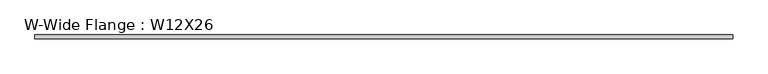
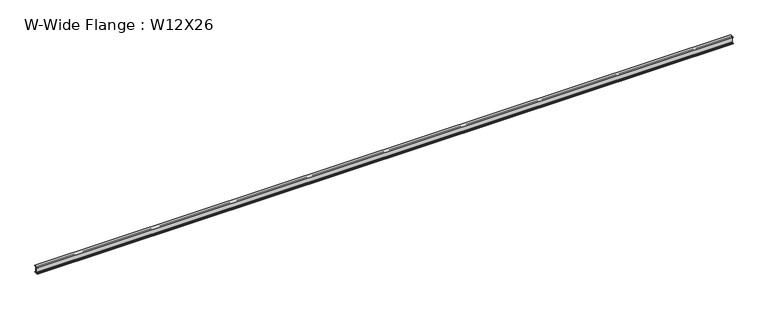
"""IFC4 building model written with IfcOpenShell, lengths in millimetres: beam geometry, W-Wide Flange : W12X26."""

import ifcopenshell
import ifcopenshell.guid

model = None  # the IFC model being written
_history = None  # IfcOwnerHistory: only IFC2X3 demands one
_inside = {}  # id of a spatial element -> (the spatial element, [elements in it])
_under = {}  # id of a project, library or spatial element -> (it, [spatial elements below it])
_declared = {}  # id of a project -> (the project, [libraries it declares])
_typed = {}  # id of a type object -> (the type object, [elements of that type])
_made_of = {}  # id of a material, layer set ... -> (it, [elements and type objects made of it])


def new_model(schema):
    """Start an empty IFC model of exactly this schema.

    Asked for "IFC4X3", IfcOpenShell would pick the latest addendum, in which some entities
    have other attributes; the version numbers below select the first issue.
    IFC2X3 requires an IfcOwnerHistory on every rooted entity: one is made here for all.
    """
    global model, _history
    if schema == "IFC4X3":
        model = ifcopenshell.file(schema_version=(4, 3, 0, 0))
    else:
        model = ifcopenshell.file(schema=schema)
    _inside.clear()
    _under.clear()
    _declared.clear()
    _typed.clear()
    _made_of.clear()
    _history = None
    if model.schema == "IFC2X3":
        org = make("IfcOrganization", Name="unknown")
        user = make(
            "IfcPersonAndOrganization",
            ThePerson=make("IfcPerson", FamilyName="unknown"),
            TheOrganization=org,
        )
        app = make(
            "IfcApplication",
            ApplicationDeveloper=org,
            Version="unknown",
            ApplicationFullName="unknown",
            ApplicationIdentifier="unknown",
        )
        _history = make(
            "IfcOwnerHistory",
            OwningUser=user,
            OwningApplication=app,
            ChangeAction="ADDED",
            CreationDate=0,
        )
    return model


def make(cls, **values):
    """One entity of the class cls with the attributes given. An attribute that is None is left unset."""
    return model.create_entity(
        cls, **{name: value for name, value in values.items() if value is not None}
    )


def rooted(cls, **values):
    """An entity with a GlobalId (a new one), such as an element, a storey or a relation."""
    return make(cls, GlobalId=ifcopenshell.guid.new(), OwnerHistory=_history, **values)


def si_unit(unit_type, name, prefix=None):
    """IfcSIUnit, for example si_unit("LENGTHUNIT", "METRE", prefix="MILLI")."""
    return make("IfcSIUnit", UnitType=unit_type, Prefix=prefix, Name=name)


def assignment(units):
    """IfcUnitAssignment: the units of a project."""
    return None if units is None else make("IfcUnitAssignment", Units=units)


def point(xyz):
    """IfcCartesianPoint."""
    return None if xyz is None else make("IfcCartesianPoint", Coordinates=xyz)


def direction(xyz):
    """IfcDirection."""
    return None if xyz is None else make("IfcDirection", DirectionRatios=xyz)


def frame(location, z_axis=None, x_axis=None):
    """IfcAxis2Placement3D, a coordinate frame: its origin and axes. An axis left out is left unset."""
    return make(
        "IfcAxis2Placement3D",
        Location=point(location),
        Axis=direction(z_axis),
        RefDirection=direction(x_axis),
    )


def frame_2d(location, x_axis=None):
    """IfcAxis2Placement2D, a coordinate frame in the plane: its origin and x axis."""
    return make(
        "IfcAxis2Placement2D", Location=point(location), RefDirection=direction(x_axis)
    )


def origin():
    """The frame at (0, 0, 0) with its axes left unset."""
    return frame((0.0, 0.0, 0.0))


def place(relative_to, where):
    """IfcLocalPlacement: puts the frame where relative to a parent placement (None: the world)."""
    return make(
        "IfcLocalPlacement", PlacementRelTo=relative_to, RelativePlacement=where
    )


def context(
    kind, dimensions, precision=None, world=None, true_north=None, identifier=None
):
    """IfcGeometricRepresentationContext, for example the 3D "Model" context."""
    return make(
        "IfcGeometricRepresentationContext",
        ContextIdentifier=identifier,
        ContextType=kind,
        CoordinateSpaceDimension=dimensions,
        Precision=precision,
        WorldCoordinateSystem=world,
        TrueNorth=true_north,
    )


def project(units=None, contexts=None):
    """IfcProject with its units and contexts."""
    return rooted(
        "IfcProject",
        Name="project",
        RepresentationContexts=contexts,
        UnitsInContext=assignment(units),
    )


def spatial(cls, under=None, at=None, **own):
    """A site, building, storey or space (cls), placed at a placement, below another one or the project."""
    s = rooted(cls, ObjectPlacement=at, **own)
    if under is not None:
        _under.setdefault(under.id(), (under, []))[1].append(s)
    return s


def polyline(points):
    """IfcPolyline through the points."""
    return make("IfcPolyline", Points=[point(p) for p in points])


def circle_curve(where, radius):
    """IfcCircle in the frame where."""
    return make("IfcCircle", Position=where, Radius=radius)


def trimmed(basis, trim1, trim2, sense, master):
    """IfcTrimmedCurve: the piece of a basis curve between two trims."""
    return make(
        "IfcTrimmedCurve",
        BasisCurve=basis,
        Trim1=trim1,
        Trim2=trim2,
        SenseAgreement=sense,
        MasterRepresentation=master,
    )


def segment(curve, same_sense, transition):
    """IfcCompositeCurveSegment."""
    return make(
        "IfcCompositeCurveSegment",
        Transition=transition,
        SameSense=same_sense,
        ParentCurve=curve,
    )


def composite_curve(segments, self_intersect=None):
    """IfcCompositeCurve: segments joined end to end."""
    return make("IfcCompositeCurve", Segments=segments, SelfIntersect=self_intersect)


def outline(outer, holes=None, kind="AREA"):
    """IfcArbitraryClosedProfileDef: a profile drawn as a closed curve; with holes, ...WithVoids."""
    if holes is None:
        return make("IfcArbitraryClosedProfileDef", ProfileType=kind, OuterCurve=outer)
    return make(
        "IfcArbitraryProfileDefWithVoids",
        ProfileType=kind,
        OuterCurve=outer,
        InnerCurves=holes,
    )


def extrude(swept, where, along, depth):
    """IfcExtrudedAreaSolid: the profile swept, set in the frame where, extruded along a direction by depth."""
    return make(
        "IfcExtrudedAreaSolid",
        SweptArea=swept,
        Position=where,
        ExtrudedDirection=direction(along),
        Depth=depth,
    )


def shape(context_of_items, identifier, shape_type, items):
    """IfcShapeRepresentation: the items that make up one representation, for example the "Body"."""
    return make(
        "IfcShapeRepresentation",
        ContextOfItems=context_of_items,
        RepresentationIdentifier=identifier,
        RepresentationType=shape_type,
        Items=items,
    )


def source(mapping_origin, context_of_items, identifier, shape_type, items):
    """IfcRepresentationMap: a shape defined once, which mapped items show again and again."""
    return make(
        "IfcRepresentationMap",
        MappingOrigin=mapping_origin,
        MappedRepresentation=shape(context_of_items, identifier, shape_type, items),
    )


def transform(
    local_origin,
    x_axis=None,
    y_axis=None,
    z_axis=None,
    scale=None,
    scale2=None,
    scale3=None,
    uniform=True,
):
    """IfcCartesianTransformationOperator3D, or its non-uniform kind. x_axis, y_axis, z_axis: its Axis1, 2, 3."""
    if uniform:
        return make(
            "IfcCartesianTransformationOperator3D",
            Axis1=direction(x_axis),
            Axis2=direction(y_axis),
            LocalOrigin=point(local_origin),
            Scale=scale,
            Axis3=direction(z_axis),
        )
    return make(
        "IfcCartesianTransformationOperator3DnonUniform",
        Axis1=direction(x_axis),
        Axis2=direction(y_axis),
        LocalOrigin=point(local_origin),
        Scale=scale,
        Axis3=direction(z_axis),
        Scale2=scale2,
        Scale3=scale3,
    )


def mapped(mapping_source, mapping_target):
    """IfcMappedItem: shows the shape of a source again, moved by a transform."""
    return make(
        "IfcMappedItem", MappingSource=mapping_source, MappingTarget=mapping_target
    )


def made_of(thing, what):
    """Note that an element or type object is made of a material, layer set ...; save() writes the relation."""
    if what is not None:
        _made_of.setdefault(what.id(), (what, []))[1].append(thing)
    return thing


def element(
    cls,
    number,
    at=None,
    inside=None,
    cuts=None,
    type_object=None,
    material=None,
    context=None,
    identifier="Body",
    shape_type=None,
    held_by="IfcProductDefinitionShape",
    body=None,
    shapes=None,
    **own,
):
    """One element of the class cls, such as IfcWall. Its Tag is "e" and its number.

    at: its placement. inside: the storey or other place that contains it. cuts: it is an
    opening in that element (IfcRelVoidsElement). A single representation is given by context,
    identifier, shape_type and body (its items); several are given by shapes. held_by: the class
    of the entity that holds the representations. save() writes the other relations.
    """
    e = rooted(cls, Tag="e%d" % number, ObjectPlacement=at, **own)
    if body is not None:
        shapes = [shape(context, identifier, shape_type, body)]
    if shapes is not None:
        e.Representation = make(held_by, Representations=shapes)
    if inside is not None:
        _inside.setdefault(inside.id(), (inside, []))[1].append(e)
    if cuts is not None:
        rooted(
            "IfcRelVoidsElement", RelatingBuildingElement=cuts, RelatedOpeningElement=e
        )
    if type_object is not None:
        _typed.setdefault(type_object.id(), (type_object, []))[1].append(e)
    return made_of(e, material)


def aggregate(whole, parts):
    """IfcRelAggregates: a whole, such as a stair, and the parts it consists of."""
    return rooted("IfcRelAggregates", RelatingObject=whole, RelatedObjects=parts)


def save(model, path):
    """Write the relations noted so far, then the file.

    IfcRelAggregates (storeys below a building ...), IfcRelContainedInSpatialStructure (elements
    in a storey), IfcRelDefinesByType, IfcRelAssociatesMaterial and IfcRelDeclares: one each for
    every whole, place, type object, material and project.
    """
    for whole, parts in _under.values():
        aggregate(whole, parts)
    for where, things in _inside.values():
        rooted(
            "IfcRelContainedInSpatialStructure",
            RelatedElements=things,
            RelatingStructure=where,
        )
    for kind, things in _typed.values():
        rooted("IfcRelDefinesByType", RelatedObjects=things, RelatingType=kind)
    for what, things in _made_of.values():
        rooted("IfcRelAssociatesMaterial", RelatedObjects=things, RelatingMaterial=what)
    for by, libraries in _declared.values():
        rooted("IfcRelDeclares", RelatingContext=by, RelatedDefinitions=libraries)
    model.write(path)


def w_wide_flange_w12x26_ee37c196(model_context):
    return source(origin(), model_context, "Body", "SweptSolid", [
        extrude(outline(composite_curve([segment(polyline([(82.4011719, -145.5539063), (82.4011719, -155.178125), (-82.4011719, -155.178125), (-82.4011719, -145.5539063), (-20.2902344, -145.5539063)]), True, "CONTINUOUS"), segment(trimmed(circle_curve(frame_2d((-20.2902344, -128.190625)), 17.3632812), [point((-20.2902344, -145.5539063))], [point((-2.9269531, -128.190625))], True, "CARTESIAN"), True, "CONTINUOUS"), segment(polyline([(-2.9269531, -128.190625), (-2.9269531, 128.190625)]), True, "CONTINUOUS"), segment(trimmed(circle_curve(frame_2d((-20.2902344, 128.190625)), 17.3632812), [point((-2.9269531, 128.190625))], [point((-20.2902344, 145.5539062))], True, "CARTESIAN"), True, "CONTINUOUS"), segment(polyline([(-20.2902344, 145.5539062), (-82.4011719, 145.5539062), (-82.4011719, 155.178125), (82.4011719, 155.178125), (82.4011719, 145.5539062), (20.2902344, 145.5539062)]), True, "CONTINUOUS"), segment(trimmed(circle_curve(frame_2d((20.2902344, 128.190625)), 17.3632812), [point((20.2902344, 145.5539062))], [point((2.9269531, 128.190625))], True, "CARTESIAN"), True, "CONTINUOUS"), segment(polyline([(2.9269531, 128.190625), (2.9269531, -128.190625)]), True, "CONTINUOUS"), segment(trimmed(circle_curve(frame_2d((20.2902344, -128.190625)), 17.3632812), [point((2.9269531, -128.190625))], [point((20.2902344, -145.5539063))], True, "CARTESIAN"), True, "CONTINUOUS"), segment(polyline([(20.2902344, -145.5539063), (82.4011719, -145.5539063)]), True, "CONTINUOUS")], self_intersect=False)), frame((-15621.0, 0.0, 0.0), z_axis=(1.0, 0.0, 0.0), x_axis=(0.0, 1.0, 0.0)), (0.0, 0.0, 1.0), 31242.0),
    ])


if __name__ == "__main__":
    model = new_model("IFC4")
    model_context = context("Model", 3, world=origin())
    ifc_project = project(units=[si_unit("LENGTHUNIT", "METRE", prefix="MILLI")], contexts=[model_context])
    site = spatial("IfcSite", under=ifc_project)
    building = spatial("IfcBuilding", under=site)
    placement = place(None, origin())
    w_wide_flange_w12x26_shape = w_wide_flange_w12x26_ee37c196(model_context)
    element("IfcBeam", 1, ObjectType="W-Wide Flange : W12X26", at=placement, inside=building, context=model_context, shape_type="MappedRepresentation", body=[
        mapped(w_wide_flange_w12x26_shape, transform((0.0, 0.0, 0.0), x_axis=(1.0, 0.0, 0.0), y_axis=(0.0, 1.0, 0.0), z_axis=(0.0, 0.0, 1.0))),
    ])
    save(model, "model.ifc")

# Revit data of these elements
# Type "W-Wide Flange : W12X26"
#   Assembly Code = "B10"
#   W = 26
#   Length [instance default] = 5' - 0"
#   bf = 0' - 6 125/256"
#   d = 1' - 0 7/32"
#   k = 0' - 1 1/16"
#   k2 = 0' - 0 175/256"
#   tf = 0' - 0 97/256"
#   tw = 0' - 0 59/256"
#   A = 0.053125 SF
#   Structural Material [instance default] = none
